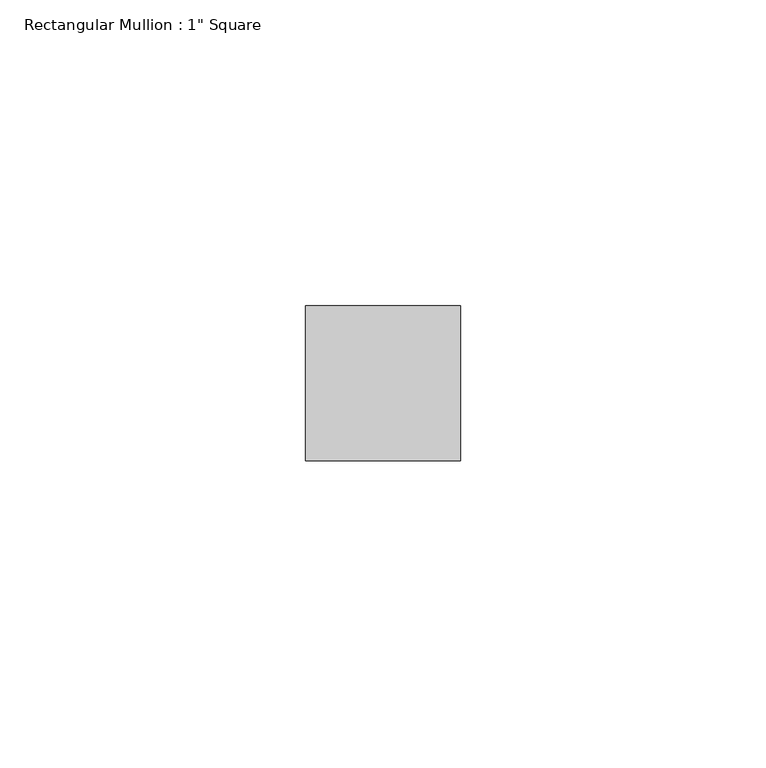
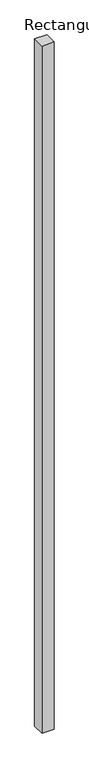
"""IFC4 building model written with IfcOpenShell, lengths in millimetres: member geometry."""

from ifc_helpers import new_model, si_unit, frame, origin, place, context, project, spatial, polyline, outline, extrude, source, transform, mapped, element, save


def member_13ff82b4(model_context):
    return source(origin(), model_context, "Body", "SweptSolid", [
        extrude(outline(polyline([(12.7, 12.7), (12.7, -12.7), (-12.7, -12.7), (-12.7, 12.7), (12.7, 12.7)])), frame((0.0, 0.0, -1498.6000003), z_axis=(0.0, 0.0, 1.0), x_axis=(1.0, 0.0, 0.0)), (0.0, 0.0, 1.0), 1498.6000003),
    ])


if __name__ == "__main__":
    model = new_model("IFC4")
    model_context = context("Model", 3, world=origin())
    ifc_project = project(units=[si_unit("LENGTHUNIT", "METRE", prefix="MILLI")], contexts=[model_context])
    site = spatial("IfcSite", under=ifc_project)
    building = spatial("IfcBuilding", under=site)
    placement = place(None, origin())
    member_shape = member_13ff82b4(model_context)
    element("IfcMember", 1, ObjectType="Rectangular Mullion : 1\" Square", at=placement, inside=building, context=model_context, shape_type="MappedRepresentation", body=[
        mapped(member_shape, transform((0.0, 0.0, 0.0), x_axis=(1.0, 0.0, 0.0), y_axis=(0.0, 1.0, 0.0), z_axis=(0.0, 0.0, 1.0))),
    ])
    save(model, "model.ifc")

# Revit data of these elements
# Type "Rectangular Mullion : 1\" Square"
#   built-in parameter 1007304 = 0.0833333 (stored number, unit not read)
#   built-in parameter 1007301 = 0.0416667 (stored number, unit not read)
#   built-in parameter 1007300 = 0.0416667 (stored number, unit not read)
# Element 1 (IfcMember, "Rectangular Mullion : 1\" Square")
#   Materials on its faces: "Metal - Aluminum"
# Materials
#   "Metal - Aluminum": class "Metal", colour RGB 247 247 247, transparency 0
